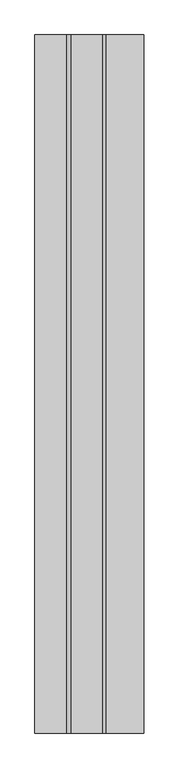
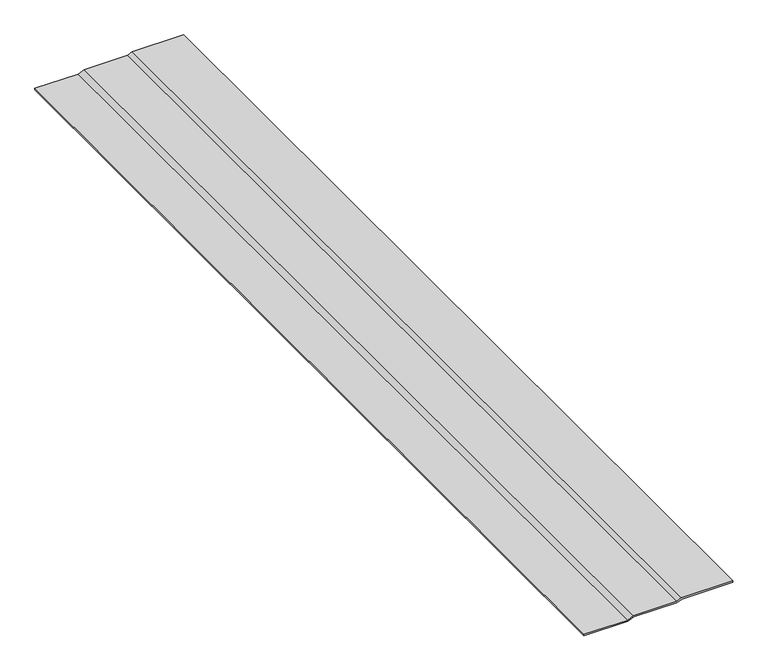
"""IFC4 building model written with IfcOpenShell, lengths in millimetres: proxy geometry, BITUMEN CAP SHEET002 3836 : BITUMEN CAP SHEET002 3836."""

from ifc_helpers import new_model, si_unit, frame, origin, place, context, project, spatial, polyline, outline, extrude, source, transform, mapped, element, save


def generic_models_cc5fe4d3(model_context):
    return source(origin(), model_context, "Body", "SweptSolid", [
        extrude(outline(polyline([(40259.2002678, -4699.8063764), (40259.2002678, -4607.6417148), (40264.4862773, -4595.1768962), (40264.4862773, -4504.46274), (40268.8188423, -4494.7463535), (40268.8188423, -4387.5351424), (40271.9940719, -4387.5351424), (40271.9940719, -4495.421639), (40267.6612773, -4505.1385405), (40267.6612773, -4595.8222961), (40262.3752678, -4608.2871148), (40262.3752678, -4699.8063764), (40259.2002678, -4699.8063764)])), frame((0.0, -1052.8906574, 0.0), z_axis=(0.0, 1.0, 0.0), x_axis=(0.0, 0.0, 1.0)), (0.0, 0.0, 1.0), 2000.25),
    ])


if __name__ == "__main__":
    model = new_model("IFC4")
    model_context = context("Model", 3, world=origin())
    ifc_project = project(units=[si_unit("LENGTHUNIT", "METRE", prefix="MILLI")], contexts=[model_context])
    site = spatial("IfcSite", under=ifc_project)
    building = spatial("IfcBuilding", under=site)
    placement = place(None, origin())
    generic_models_shape = generic_models_cc5fe4d3(model_context)
    element("IfcBuildingElementProxy", 1, Name="BITUMEN CAP SHEET002 3836 : BITUMEN CAP SHEET002 3836", ObjectType="BITUMEN CAP SHEET002 3836 : BITUMEN CAP SHEET002 3836", at=placement, inside=building, context=model_context, shape_type="MappedRepresentation", body=[
        mapped(generic_models_shape, transform((0.0, 0.0, 0.0), x_axis=(1.0, 0.0, 0.0), y_axis=(0.0, 1.0, 0.0), z_axis=(0.0, 0.0, 1.0))),
    ])
    save(model, "model.ifc")

# Revit data of these elements
# Type "BITUMEN CAP SHEET002 3836 : BITUMEN CAP SHEET002 3836"
#   NameOverride = "BITUMEN CAP SHEET002"
# Element 1 (IfcBuildingElementProxy, "BITUMEN CAP SHEET002 3836 : BITUMEN CAP SHEET002 3836")
#   Materials on its faces: "MODIFIED BITUMEN GRANULE SURFACED CAP SHEET"
# Materials
#   "MODIFIED BITUMEN GRANULE SURFACED CAP SHEET": class "Unassigned", colour RGB 85 85 127, transparency 0
